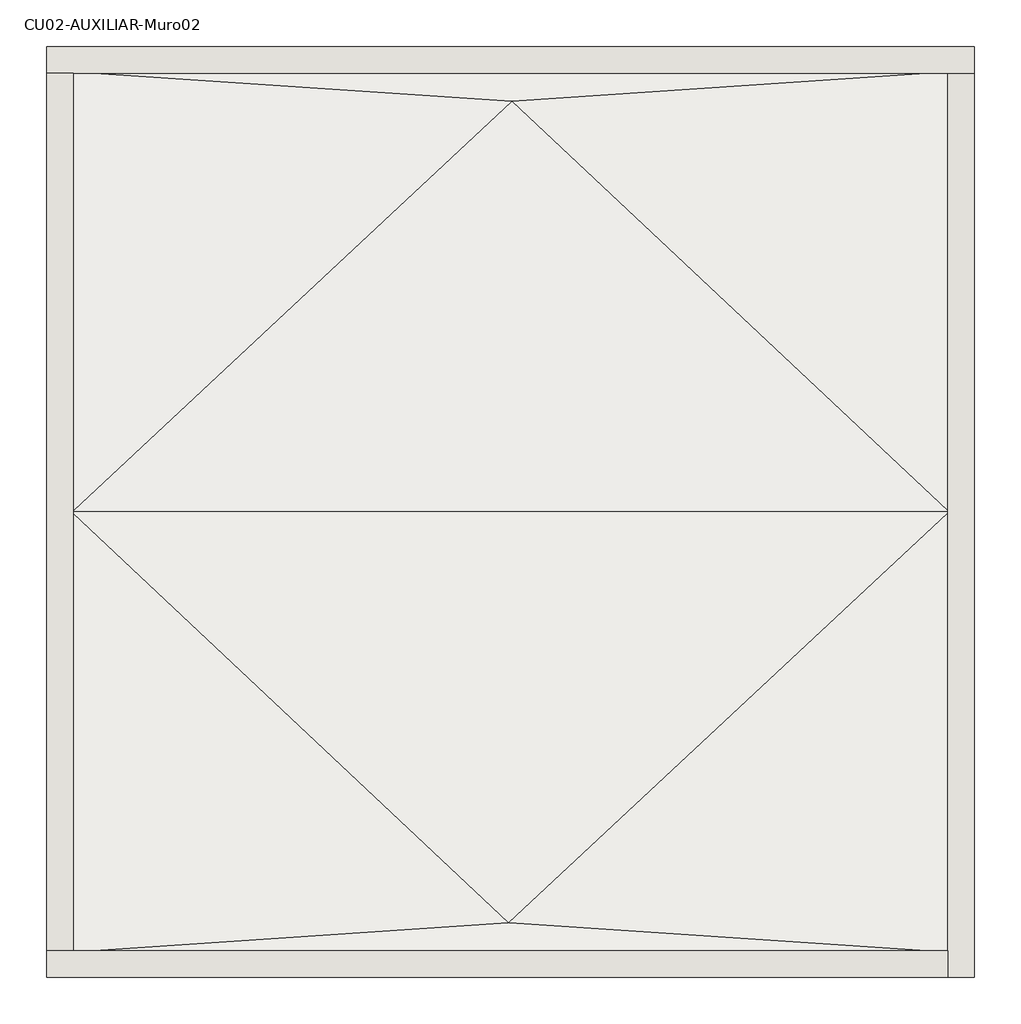
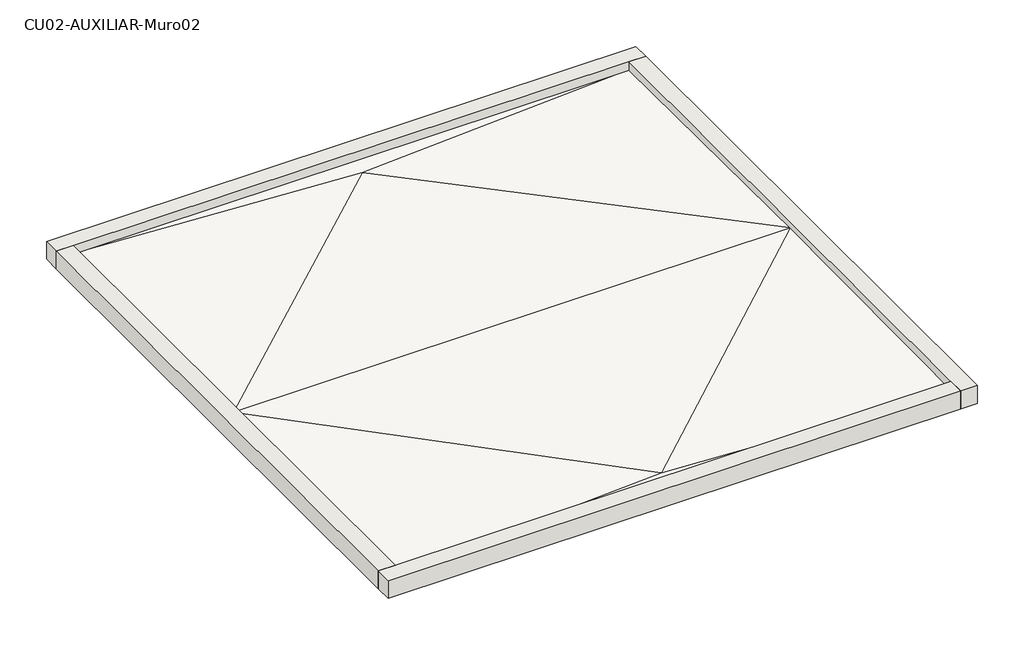
# One storey: 4 walls, 1 roof.
"""IFC4 building model written with IfcOpenShell, lengths in millimetres."""

from ifc_helpers import new_model, si_unit, origin, place, context, project, spatial, faceted_brep, element, save

model = new_model("IFC4")

# Units and contexts
model_context = context("Model", 3, world=origin())
ifc_project = project(units=[si_unit("LENGTHUNIT", "METRE", prefix="MILLI")], contexts=[model_context])

# Site, building, storey
site = spatial("IfcSite", under=ifc_project)
building = spatial("IfcBuilding", under=site)
storey = spatial("IfcBuildingStorey", under=building, Name="CU02-AUXILIAR-Muro02", Elevation=6850.0)

# Roof
placement = place(None, origin())
element("IfcRoof", 1, ObjectType="ACAB CUB GRAVA SUP_PABLO", at=placement, inside=storey, context=model_context, shape_type="Brep", body=[
    faceted_brep([(-20975.0, -4507.5, 6850.0), (-12025.0, -4507.5, 6850.0), (-12025.0, -4522.5, 6850.0), (-12025.0, -13492.5, 6850.0), (-12040.0, -13492.5, 6850.0), (-20975.0, -13492.5, 6850.0), (-20975.0, -13477.5, 6850.0), (-20975.0, -4522.5, 6850.0), (-12025.0, -4507.5, 7001.2), (-20975.0, -4507.5, 7001.2), (-16482.5, -4507.5, 7001.2), (-20975.0, -13492.5, 7001.2), (-20975.0, -13477.5, 7001.3335559), (-20975.0, -9000.0, 7041.2), (-20975.0, -4522.5, 7001.3335559), (-12025.0, -13492.5, 7001.2), (-12025.0, -4522.5, 7001.3335559), (-12025.0, -9000.0, 7041.2), (-12040.0, -13492.5, 7001.2), (-16517.5, -13492.5, 7001.2), (-20960.0, -8986.0122737, 7041.0443214), (-16482.5, -4810.6759755, 6994.5742457), (-20752.7281004, -4522.5, 7000.8721827), (-12040.0, -13491.4877263, 7001.1778773), (-12247.2718996, -13477.5, 7000.8721827), (-16517.5, -13189.3240245, 6994.5742457), (-20754.4597679, -13477.5, 7000.8721827), (-12040.0, -9013.9877263, 7041.0443214), (-12040.0, -9000.0, 7041.2), (-20960.0, -9000.0, 7041.2), (-20960.0, -9014.097557, 7041.043099), (-12040.0, -8985.902443, 7041.043099), (-12245.5402321, -4522.5, 7000.8721827)], [[[0, 1, 2, 3, 4, 5, 6, 7]], [[8, 1, 0, 9, 10]], [[9, 0, 7, 6, 5, 11, 12, 13, 14]], [[15, 3, 2, 1, 8, 16, 17]], [[11, 5, 4, 3, 15, 18, 19]], [[9, 14, 13, 20, 21, 22]], [[11, 19, 18, 15, 23, 24, 25, 26]], [[15, 17, 27, 25, 24, 23]], [[17, 28, 29, 13, 30, 25, 27]], [[11, 26, 25, 30, 13, 12]], [[17, 31, 21, 20, 13, 29, 28]], [[8, 32, 21, 31, 17, 16]], [[9, 22, 21, 32, 8, 10]]]),
])

# Walls
element("IfcWall", 2, ObjectType="MURO TIPO 5_PETO CUB_PABLO", at=placement, inside=storey, context=model_context, shape_type="Brep", body=[
    faceted_brep([(-11770.0, -4522.5, 7150.0), (-12040.0, -4522.5, 7150.0), (-20960.0, -4522.5, 7150.0), (-21230.0, -4522.5, 7150.0), (-21230.0, -4522.5, 6850.0), (-20975.0, -4522.5, 6850.0), (-20975.0, -4522.5, 7001.3335559), (-20752.7281004, -4522.5, 7000.8721827), (-12245.5402321, -4522.5, 7000.8721827), (-12025.0, -4522.5, 7001.3335559), (-12025.0, -4522.5, 6850.0), (-11770.0, -4522.5, 6850.0), (-11770.0, -4252.5, 6850.0), (-21230.0, -4252.5, 6850.0), (-21230.0, -4252.5, 7150.0), (-11770.0, -4252.5, 7150.0), (-12025.0, -4507.5, 6850.0), (-20975.0, -4507.5, 6850.0), (-12025.0, -4507.5, 7001.2), (-16482.5, -4507.5, 7001.2), (-20975.0, -4507.5, 7001.2)], [[[0, 1, 2, 3, 4, 5, 6, 7, 8, 9, 10, 11]], [[12, 13, 14, 15]], [[13, 12, 11, 10, 16, 17, 5, 4]], [[3, 2, 1, 0, 15, 14]], [[0, 11, 12, 15]], [[4, 3, 14, 13]], [[16, 18, 19, 20, 17]], [[17, 20, 6, 5]], [[18, 16, 10, 9]], [[6, 20, 7]], [[18, 9, 8]], [[20, 19, 18, 8, 7]]]),
])
element("IfcWall", 3, ObjectType="MURO TIPO 5_PETO CUB_PABLO", at=placement, inside=storey, context=model_context, shape_type="Brep", body=[
    faceted_brep([(-12040.0, -13747.5, 7150.0), (-12040.0, -13477.5, 7150.0), (-12040.0, -4522.5, 7150.0), (-12040.0, -4522.5, 7001.3021757), (-12040.0, -8985.902443, 7041.043099), (-12040.0, -9000.0, 7041.2), (-12040.0, -9013.9877263, 7041.0443214), (-12040.0, -13491.4877263, 7001.1778773), (-12040.0, -13492.5, 7001.2), (-12040.0, -13492.5, 6850.0), (-12040.0, -13747.5, 6850.0), (-11770.0, -13747.5, 6850.0), (-11770.0, -4522.5, 6850.0), (-11770.0, -4522.5, 7150.0), (-11770.0, -13747.5, 7150.0), (-12025.0, -13492.5, 6850.0), (-12025.0, -4522.5, 6850.0), (-12025.0, -4522.5, 7001.3335559), (-12025.0, -13492.5, 7001.2), (-12025.0, -9000.0, 7041.2)], [[[0, 1, 2, 3, 4, 5, 6, 7, 8, 9, 10]], [[11, 12, 13, 14]], [[12, 11, 10, 9, 15, 16]], [[2, 1, 0, 14, 13]], [[2, 13, 12, 16, 17, 3]], [[0, 10, 11, 14]], [[15, 18, 19, 17, 16]], [[18, 15, 9, 8]], [[19, 18, 7, 6]], [[5, 19, 6]], [[18, 8, 7]], [[19, 5, 4]], [[17, 19, 4, 3]]]),
])
element("IfcWall", 4, ObjectType="MURO TIPO 5_PETO CUB_PABLO", at=placement, inside=storey, context=model_context, shape_type="Brep", body=[
    faceted_brep([(-21230.0, -13477.5, 7150.0), (-20960.0, -13477.5, 7150.0), (-12040.0, -13477.5, 7150.0), (-12040.0, -13477.5, 7001.3024202), (-12247.2718996, -13477.5, 7000.8721827), (-20754.4597679, -13477.5, 7000.8721827), (-20975.0, -13477.5, 7001.3335559), (-20975.0, -13477.5, 6850.0), (-21230.0, -13477.5, 6850.0), (-21230.0, -13747.5, 6850.0), (-12040.0, -13747.5, 6850.0), (-12040.0, -13747.5, 7150.0), (-21230.0, -13747.5, 7150.0), (-20975.0, -13492.5, 6850.0), (-12040.0, -13492.5, 6850.0), (-12040.0, -13492.5, 7001.2), (-12040.0, -13491.4877263, 7001.1778773), (-20975.0, -13492.5, 7001.2), (-16517.5, -13492.5, 7001.2)], [[[0, 1, 2, 3, 4, 5, 6, 7, 8]], [[9, 10, 11, 12]], [[10, 9, 8, 7, 13, 14]], [[2, 1, 0, 12, 11]], [[2, 11, 10, 14, 15, 16, 3]], [[0, 8, 9, 12]], [[17, 13, 7, 6]], [[13, 17, 18, 15, 14]], [[18, 17, 5, 4, 16, 15]], [[4, 3, 16]], [[17, 6, 5]]]),
])
element("IfcWall", 5, ObjectType="MURO TIPO 5_PETO CUB_PABLO", at=placement, inside=storey, context=model_context, shape_type="Brep", body=[
    faceted_brep([(-20960.0, -4522.5, 7150.0), (-20960.0, -13477.5, 7150.0), (-20960.0, -13477.5, 7001.3021757), (-20960.0, -9014.097557, 7041.043099), (-20960.0, -9000.0, 7041.2), (-20960.0, -8986.0122737, 7041.0443214), (-20960.0, -4522.5, 7001.3024202), (-21230.0, -4522.5, 6850.0), (-21230.0, -13477.5, 6850.0), (-21230.0, -13477.5, 7150.0), (-21230.0, -4522.5, 7150.0), (-20975.0, -4522.5, 6850.0), (-20975.0, -13477.5, 6850.0), (-20975.0, -13477.5, 7001.3335559), (-20975.0, -4522.5, 7001.3335559), (-20975.0, -9000.0, 7041.2)], [[[0, 1, 2, 3, 4, 5, 6]], [[7, 8, 9, 10]], [[8, 7, 11, 12]], [[1, 0, 10, 9]], [[1, 9, 8, 12, 13, 2]], [[7, 10, 0, 6, 14, 11]], [[12, 11, 14, 15, 13]], [[15, 14, 6, 5]], [[15, 4, 3]], [[13, 15, 3, 2]], [[4, 15, 5]]]),
])

save(model, "model.ifc")

# Revit data of these elements
# Type "ACAB CUB GRAVA SUP_PABLO"
#   Keynote = ""
#   Layers, outside or top first: 0.05 m "Grava capa acabado" (function 4); 0.00 m "Geotextil capa separadora" (function 100); 0.04 m "Poliestireno extruido (XPS)" (function 3); 0.0012 m "Membrana impermeabilizante" (function 3); 0.00 m "Geotextil capa separadora" (function 100); 0.10 m "Hormigón celular" (function 2)
# Type "MURO TIPO 5_PETO CUB_PABLO"
#   Keynote = "Md.1"
#   Description = "Muro interior-interior patio exterior"
#   Type Mark = "M5"
#   Layers, outside or top first: 0.015 m "Enfoscado cemento y pintura" (function 5); 0.24 m "Ladrillo cerámico perforado" (function 1); 0.015 m "Enfoscado cemento y pintura" (function 5)
# Element 1 (IfcRoof, "ACAB CUB GRAVA SUP_PABLO")
#   built-in parameter 1001705 = 23.101 (stored number, unit not read)
#   built-in parameter 1001701 = 0 (stored number, unit not read)
#   built-in parameter 1001710 = 33615
#   Phase Created = Nueva construcción
#   Materials on its faces: "Grava capa acabado", "Hormigón celular"
# Elements 2, 3, 4, 5 (IfcWall, "MURO TIPO 5_PETO CUB_PABLO")
#   Top Offset = 0.00 m
#   Base Offset = 0.00 m
#   wall height = 0.30 m
#   Phase Created = Nueva construcción
#   Base Constraint = CU02-AUXILIAR-Muro02
#   Top Constraint = AUXILIAR-CoronacionMuro
#   Materials on its faces: "Muro por defecto", "Enfoscado cemento y pintura"
# Materials
#   "Grava capa acabado": class "Varios", colour RGB 0 0 0, transparency 0, Comments = "Canto rodado 5 cm espesor medio", Cost = 0
#   "Geotextil capa separadora": class "Plástico", colour RGB 127 127 127, transparency 0, Comments = "Fieltro sintético fe\nltemper", Description = "Acabado exterior, cubierta", Cost = 0
#   "Poliestireno extruido (XPS)": class "Plástico", colour RGB 120 120 120, transparency 0, Comments = "Aislamiento térmico de célula cerrada", Description = "Plancha de poliestireno extruido", Cost = 0
#   "Membrana impermeabilizante": class "Plástico", colour RGB 127 127 127, transparency 0, Comments = "Lámina (1,2 mm) armada con fibra de vidrio", Description = "Acabado exterior, cubierta", Cost = 0
#   "Hormigón celular": class "Hormigón", colour RGB 120 120 120, transparency 0, Comments = "Capa de formación de pte", Description = "Hormigón ligero", Cost = 0
#   "Enfoscado cemento y pintura": class "Varios", colour RGB 127 127 127, transparency 0, Keynote = "2", Comments = "Color blanco (1,5 cm)", Cost = 0
#   "Ladrillo cerámico perforado": class "Enladrillado", colour RGB 204 146 111, transparency 0, Cost = 0
#   "Muro por defecto": class "Varios", colour RGB 212 212 212, transparency 0, Cost = 0
